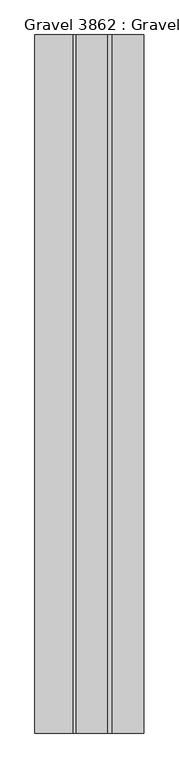
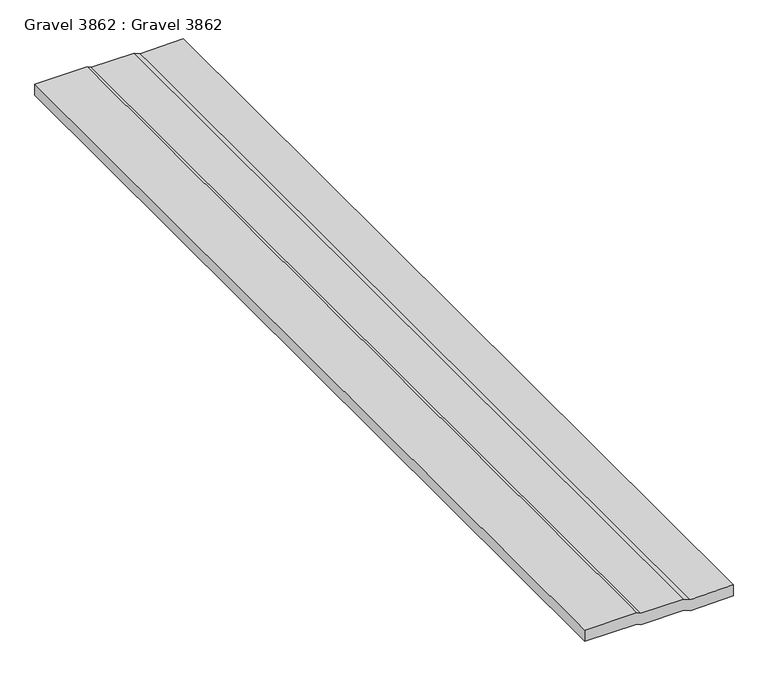
"""IFC4 building model written with IfcOpenShell, lengths in millimetres: proxy geometry, Gravel 3862 : Gravel 3862."""

from ifc_helpers import new_model, si_unit, frame, origin, place, context, project, spatial, polyline, outline, extrude, source, transform, mapped, element, save


def gravel_3862_gravel_3862_052f081c(model_context):
    return source(origin(), model_context, "Body", "SweptSolid", [
        extrude(outline(polyline([(40274.2359464, -4902.3767758), (40269.9546964, -4893.6663265), (40269.9546964, -4803.0794125), (40264.2272344, -4790.2347731), (40265.8726651, -4699.8063764), (40290.6109464, -4699.8063764), (40288.9655157, -4790.2347731), (40294.6929777, -4803.0794125), (40294.6929777, -4893.6663265), (40298.9742277, -4902.3767758), (40298.9742277, -5011.8762875), (40274.2359464, -5011.8762875), (40274.2359464, -4902.3767758)])), frame((0.0, -1052.6406573, 0.0), z_axis=(0.0, 1.0, 0.0), x_axis=(0.0, 0.0, 1.0)), (0.0, 0.0, 1.0), 2000.0),
    ])


if __name__ == "__main__":
    model = new_model("IFC4")
    model_context = context("Model", 3, world=origin())
    ifc_project = project(units=[si_unit("LENGTHUNIT", "METRE", prefix="MILLI")], contexts=[model_context])
    site = spatial("IfcSite", under=ifc_project)
    building = spatial("IfcBuilding", under=site)
    placement = place(None, origin())
    gravel_3862_gravel_3862_shape = gravel_3862_gravel_3862_052f081c(model_context)
    element("IfcBuildingElementProxy", 1, Name="Gravel 3862 : Gravel 3862", ObjectType="Gravel 3862 : Gravel 3862", at=placement, inside=building, context=model_context, shape_type="MappedRepresentation", body=[
        mapped(gravel_3862_gravel_3862_shape, transform((0.0, 0.0, 0.0), x_axis=(1.0, 0.0, 0.0), y_axis=(0.0, 1.0, 0.0), z_axis=(0.0, 0.0, 1.0))),
    ])
    save(model, "model.ifc")

# Revit data of these elements
# Type "Gravel 3862 : Gravel 3862"
#   NameOverride = "Gravel"
# Element 1 (IfcBuildingElementProxy, "Gravel 3862 : Gravel 3862")
#   Materials on its faces: "GRAVEL BALLAST"
# Materials
#   "GRAVEL BALLAST": class "Unassigned", colour RGB 128 128 128, transparency 0, Cost = 0
